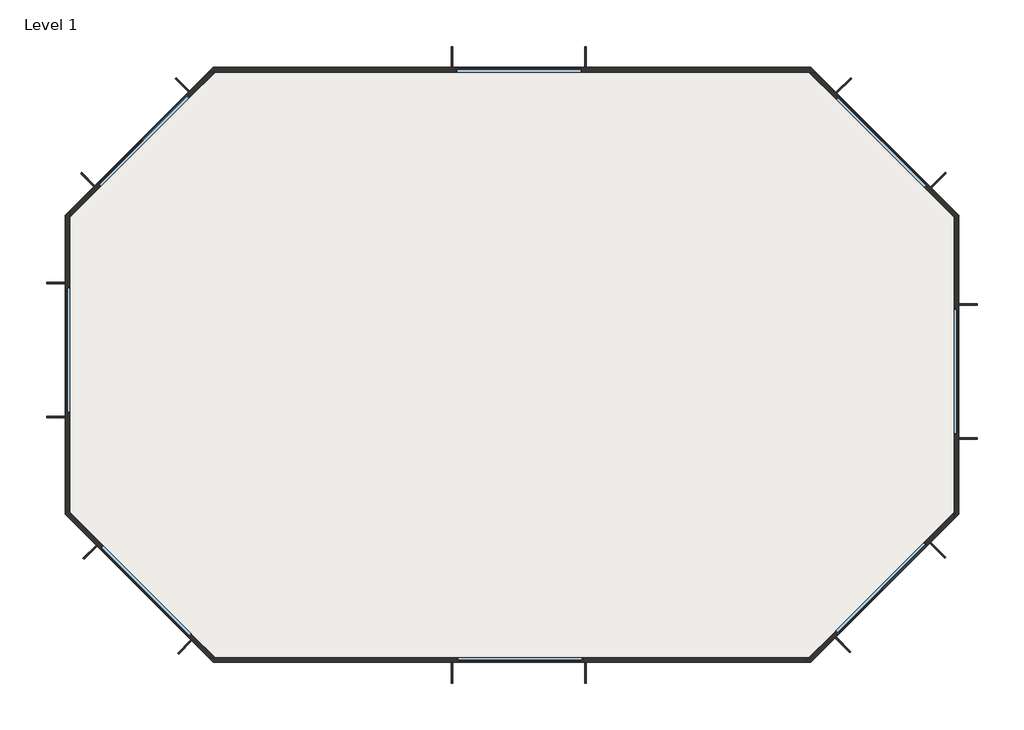
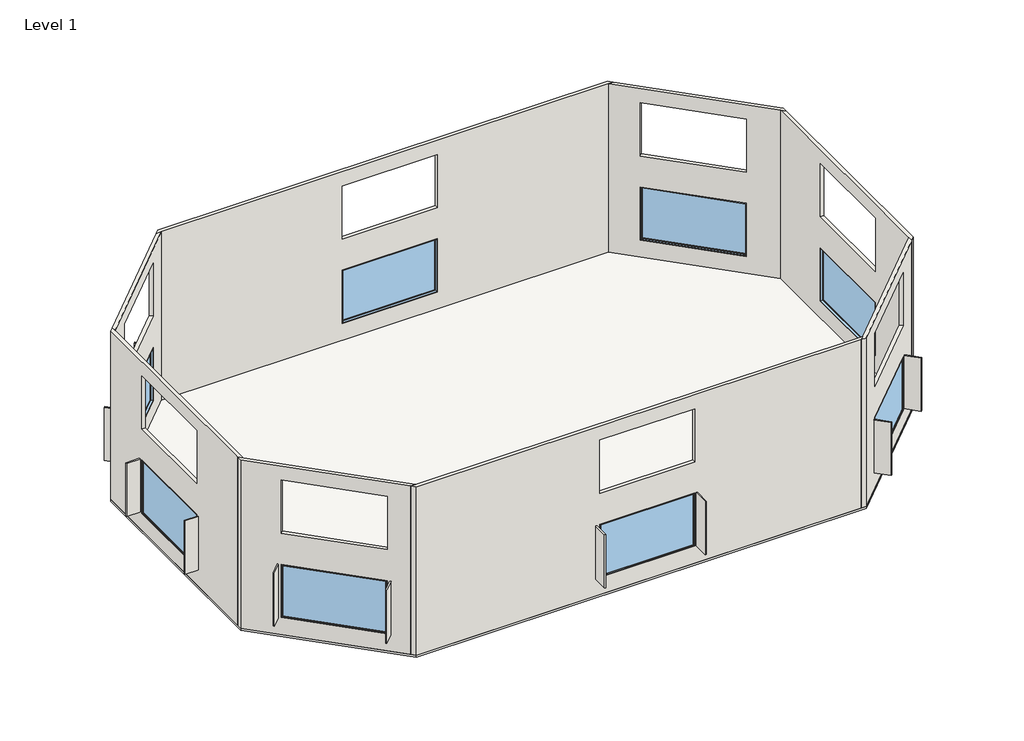
# One storey: 24 walls, 8 windows, 1 slab.
"""IFC4 building model written with IfcOpenShell, lengths in millimetres."""

import ifcopenshell
import ifcopenshell.guid

model = None  # the IFC model being written
_history = None  # IfcOwnerHistory: only IFC2X3 demands one
_inside = {}  # id of a spatial element -> (the spatial element, [elements in it])
_under = {}  # id of a project, library or spatial element -> (it, [spatial elements below it])
_declared = {}  # id of a project -> (the project, [libraries it declares])
_typed = {}  # id of a type object -> (the type object, [elements of that type])
_made_of = {}  # id of a material, layer set ... -> (it, [elements and type objects made of it])


def new_model(schema):
    """Start an empty IFC model of exactly this schema.

    Asked for "IFC4X3", IfcOpenShell would pick the latest addendum, in which some entities
    have other attributes; the version numbers below select the first issue.
    IFC2X3 requires an IfcOwnerHistory on every rooted entity: one is made here for all.
    """
    global model, _history
    if schema == "IFC4X3":
        model = ifcopenshell.file(schema_version=(4, 3, 0, 0))
    else:
        model = ifcopenshell.file(schema=schema)
    _inside.clear()
    _under.clear()
    _declared.clear()
    _typed.clear()
    _made_of.clear()
    _history = None
    if model.schema == "IFC2X3":
        org = make("IfcOrganization", Name="unknown")
        user = make(
            "IfcPersonAndOrganization",
            ThePerson=make("IfcPerson", FamilyName="unknown"),
            TheOrganization=org,
        )
        app = make(
            "IfcApplication",
            ApplicationDeveloper=org,
            Version="unknown",
            ApplicationFullName="unknown",
            ApplicationIdentifier="unknown",
        )
        _history = make(
            "IfcOwnerHistory",
            OwningUser=user,
            OwningApplication=app,
            ChangeAction="ADDED",
            CreationDate=0,
        )
    return model


def make(cls, **values):
    """One entity of the class cls with the attributes given. An attribute that is None is left unset."""
    return model.create_entity(
        cls, **{name: value for name, value in values.items() if value is not None}
    )


def rooted(cls, **values):
    """An entity with a GlobalId (a new one), such as an element, a storey or a relation."""
    return make(cls, GlobalId=ifcopenshell.guid.new(), OwnerHistory=_history, **values)


def si_unit(unit_type, name, prefix=None):
    """IfcSIUnit, for example si_unit("LENGTHUNIT", "METRE", prefix="MILLI")."""
    return make("IfcSIUnit", UnitType=unit_type, Prefix=prefix, Name=name)


def assignment(units):
    """IfcUnitAssignment: the units of a project."""
    return None if units is None else make("IfcUnitAssignment", Units=units)


def point(xyz):
    """IfcCartesianPoint."""
    return None if xyz is None else make("IfcCartesianPoint", Coordinates=xyz)


def direction(xyz):
    """IfcDirection."""
    return None if xyz is None else make("IfcDirection", DirectionRatios=xyz)


def frame(location, z_axis=None, x_axis=None):
    """IfcAxis2Placement3D, a coordinate frame: its origin and axes. An axis left out is left unset."""
    return make(
        "IfcAxis2Placement3D",
        Location=point(location),
        Axis=direction(z_axis),
        RefDirection=direction(x_axis),
    )


def origin():
    """The frame at (0, 0, 0) with its axes left unset."""
    return frame((0.0, 0.0, 0.0))


def place(relative_to, where):
    """IfcLocalPlacement: puts the frame where relative to a parent placement (None: the world)."""
    return make(
        "IfcLocalPlacement", PlacementRelTo=relative_to, RelativePlacement=where
    )


def context(
    kind, dimensions, precision=None, world=None, true_north=None, identifier=None
):
    """IfcGeometricRepresentationContext, for example the 3D "Model" context."""
    return make(
        "IfcGeometricRepresentationContext",
        ContextIdentifier=identifier,
        ContextType=kind,
        CoordinateSpaceDimension=dimensions,
        Precision=precision,
        WorldCoordinateSystem=world,
        TrueNorth=true_north,
    )


def project(units=None, contexts=None):
    """IfcProject with its units and contexts."""
    return rooted(
        "IfcProject",
        Name="project",
        RepresentationContexts=contexts,
        UnitsInContext=assignment(units),
    )


def spatial(cls, under=None, at=None, **own):
    """A site, building, storey or space (cls), placed at a placement, below another one or the project."""
    s = rooted(cls, ObjectPlacement=at, **own)
    if under is not None:
        _under.setdefault(under.id(), (under, []))[1].append(s)
    return s


def polyline(points):
    """IfcPolyline through the points."""
    return make("IfcPolyline", Points=[point(p) for p in points])


def outline(outer, holes=None, kind="AREA"):
    """IfcArbitraryClosedProfileDef: a profile drawn as a closed curve; with holes, ...WithVoids."""
    if holes is None:
        return make("IfcArbitraryClosedProfileDef", ProfileType=kind, OuterCurve=outer)
    return make(
        "IfcArbitraryProfileDefWithVoids",
        ProfileType=kind,
        OuterCurve=outer,
        InnerCurves=holes,
    )


def extrude(swept, where, along, depth):
    """IfcExtrudedAreaSolid: the profile swept, set in the frame where, extruded along a direction by depth."""
    return make(
        "IfcExtrudedAreaSolid",
        SweptArea=swept,
        Position=where,
        ExtrudedDirection=direction(along),
        Depth=depth,
    )


def faces_of(points, faces, orient=None, outer=None):
    """IfcFace entities. A face is a list of loops; a loop is a list of indices into points, from 0.

    orient and outer hold one flag for each loop. By default every Orientation is true, the
    first loop of a face is its IfcFaceOuterBound and the others are IfcFaceBound.
    """
    made = []
    for i, loops in enumerate(faces):
        bounds = []
        for j, loop in enumerate(loops):
            is_outer = j == 0 if outer is None else outer[i][j]
            bounds.append(
                make(
                    "IfcFaceOuterBound" if is_outer else "IfcFaceBound",
                    Bound=make("IfcPolyLoop", Polygon=[points[k] for k in loop]),
                    Orientation=True if orient is None else orient[i][j],
                )
            )
        made.append(make("IfcFace", Bounds=bounds))
    return made


def faceted_brep(points, faces, orient=None, outer=None, voids=None):
    """IfcFacetedBrep: a solid bounded by flat faces; with voids (closed shells), ...WithVoids."""
    shared = [point(p) for p in points]
    hull = make("IfcClosedShell", CfsFaces=faces_of(shared, faces, orient, outer))
    if voids is None:
        return make("IfcFacetedBrep", Outer=hull)
    return make(
        "IfcFacetedBrepWithVoids",
        Outer=hull,
        Voids=[
            make(cls, CfsFaces=faces_of(shared, fs, o, b)) for cls, fs, o, b in voids
        ],
    )


def shape(context_of_items, identifier, shape_type, items):
    """IfcShapeRepresentation: the items that make up one representation, for example the "Body"."""
    return make(
        "IfcShapeRepresentation",
        ContextOfItems=context_of_items,
        RepresentationIdentifier=identifier,
        RepresentationType=shape_type,
        Items=items,
    )


def source(mapping_origin, context_of_items, identifier, shape_type, items):
    """IfcRepresentationMap: a shape defined once, which mapped items show again and again."""
    return make(
        "IfcRepresentationMap",
        MappingOrigin=mapping_origin,
        MappedRepresentation=shape(context_of_items, identifier, shape_type, items),
    )


def transform(
    local_origin,
    x_axis=None,
    y_axis=None,
    z_axis=None,
    scale=None,
    scale2=None,
    scale3=None,
    uniform=True,
):
    """IfcCartesianTransformationOperator3D, or its non-uniform kind. x_axis, y_axis, z_axis: its Axis1, 2, 3."""
    if uniform:
        return make(
            "IfcCartesianTransformationOperator3D",
            Axis1=direction(x_axis),
            Axis2=direction(y_axis),
            LocalOrigin=point(local_origin),
            Scale=scale,
            Axis3=direction(z_axis),
        )
    return make(
        "IfcCartesianTransformationOperator3DnonUniform",
        Axis1=direction(x_axis),
        Axis2=direction(y_axis),
        LocalOrigin=point(local_origin),
        Scale=scale,
        Axis3=direction(z_axis),
        Scale2=scale2,
        Scale3=scale3,
    )


def mapped(mapping_source, mapping_target):
    """IfcMappedItem: shows the shape of a source again, moved by a transform."""
    return make(
        "IfcMappedItem", MappingSource=mapping_source, MappingTarget=mapping_target
    )


def made_of(thing, what):
    """Note that an element or type object is made of a material, layer set ...; save() writes the relation."""
    if what is not None:
        _made_of.setdefault(what.id(), (what, []))[1].append(thing)
    return thing


def element(
    cls,
    number,
    at=None,
    inside=None,
    cuts=None,
    type_object=None,
    material=None,
    context=None,
    identifier="Body",
    shape_type=None,
    held_by="IfcProductDefinitionShape",
    body=None,
    shapes=None,
    **own,
):
    """One element of the class cls, such as IfcWall. Its Tag is "e" and its number.

    at: its placement. inside: the storey or other place that contains it. cuts: it is an
    opening in that element (IfcRelVoidsElement). A single representation is given by context,
    identifier, shape_type and body (its items); several are given by shapes. held_by: the class
    of the entity that holds the representations. save() writes the other relations.
    """
    e = rooted(cls, Tag="e%d" % number, ObjectPlacement=at, **own)
    if body is not None:
        shapes = [shape(context, identifier, shape_type, body)]
    if shapes is not None:
        e.Representation = make(held_by, Representations=shapes)
    if inside is not None:
        _inside.setdefault(inside.id(), (inside, []))[1].append(e)
    if cuts is not None:
        rooted(
            "IfcRelVoidsElement", RelatingBuildingElement=cuts, RelatedOpeningElement=e
        )
    if type_object is not None:
        _typed.setdefault(type_object.id(), (type_object, []))[1].append(e)
    return made_of(e, material)


def aggregate(whole, parts):
    """IfcRelAggregates: a whole, such as a stair, and the parts it consists of."""
    return rooted("IfcRelAggregates", RelatingObject=whole, RelatedObjects=parts)


def save(model, path):
    """Write the relations noted so far, then the file.

    IfcRelAggregates (storeys below a building ...), IfcRelContainedInSpatialStructure (elements
    in a storey), IfcRelDefinesByType, IfcRelAssociatesMaterial and IfcRelDeclares: one each for
    every whole, place, type object, material and project.
    """
    for whole, parts in _under.values():
        aggregate(whole, parts)
    for where, things in _inside.values():
        rooted(
            "IfcRelContainedInSpatialStructure",
            RelatedElements=things,
            RelatingStructure=where,
        )
    for kind, things in _typed.values():
        rooted("IfcRelDefinesByType", RelatedObjects=things, RelatingType=kind)
    for what, things in _made_of.values():
        rooted("IfcRelAssociatesMaterial", RelatedObjects=things, RelatingMaterial=what)
    for by, libraries in _declared.values():
        rooted("IfcRelDeclares", RelatingContext=by, RelatedDefinitions=libraries)
    model.write(path)


def m_fixed_2500x_4228mm_fd5e51e7(model_context):
    return source(origin(), model_context, "Body", "SweptSolid", [
        extrude(outline(polyline([(-2050.8, 54.2), (2050.8, 54.2), (2050.8, 42.2), (-2050.8, 42.2), (-2050.8, 54.2)])), frame((0.0, 0.0, 368.0), z_axis=(0.0, 0.0, 1.0), x_axis=(1.0, 0.0, 0.0)), (0.0, 0.0, 1.0), 2374.0),
        extrude(outline(polyline([(2786.0, -2094.8), (324.0, -2094.8), (324.0, 2094.8), (2786.0, 2094.8), (2786.0, -2094.8)]), holes=[polyline([(2742.0, -2050.8), (2742.0, 2050.8), (368.0, 2050.8), (368.0, -2050.8), (2742.0, -2050.8)])]), frame((0.0, 26.2, 0.0), z_axis=(0.0, 1.0, 0.0), x_axis=(0.0, 0.0, 1.0)), (0.0, 0.0, 1.0), 44.0),
        extrude(outline(polyline([(2805.0, -2113.8), (305.0, -2113.8), (305.0, 2113.8), (2805.0, 2113.8), (2805.0, -2113.8)]), holes=[polyline([(2786.0, -2094.8), (2786.0, 2094.8), (324.0, 2094.8), (324.0, -2094.8), (2786.0, -2094.8)])]), frame((0.0, 26.2, 0.0), z_axis=(0.0, 1.0, 0.0), x_axis=(0.0, 0.0, 1.0)), (0.0, 0.0, 1.0), 63.0),
        extrude(outline(polyline([(2805.0, -2113.8), (305.0, -2113.8), (305.0, 2113.8), (2805.0, 2113.8), (2805.0, -2113.8)]), holes=[polyline([(2773.0, -2081.8), (2773.0, 2081.8), (337.0, 2081.8), (337.0, -2081.8), (2773.0, -2081.8)])]), frame((0.0, -63.2, 0.0), z_axis=(0.0, 1.0, 0.0), x_axis=(0.0, 0.0, 1.0)), (0.0, 0.0, 1.0), 89.4),
    ])


model = new_model("IFC4")

# Units and contexts
model_context = context("Model", 3, world=origin())
ifc_project = project(units=[si_unit("LENGTHUNIT", "METRE", prefix="MILLI")], contexts=[model_context])

# Site, building, storey
site = spatial("IfcSite", under=ifc_project)
building = spatial("IfcBuilding", under=site)
storey = spatial("IfcBuildingStorey", under=building, Name="Level 1", Elevation=0.0)

# Slab
placement = place(None, origin())
element("IfcSlab", 1, ObjectType="Generic Floor - 100mm", at=placement, inside=storey, context=model_context, shape_type="SweptSolid", body=[
    extrude(outline(polyline([(10639.2142415, 11296.9802217), (30639.2142415, 11296.9802217), (35588.9617098, 6347.2327534), (35588.9617098, -3652.7672466), (30639.2142415, -8602.5147149), (10639.2142415, -8602.5147149), (5689.4667732, -3652.7672466), (5689.4667732, 6347.2327534), (10639.2142415, 11296.9802217)])), frame((0.0, 0.0, -100.0), z_axis=(0.0, 0.0, 1.0), x_axis=(1.0, 0.0, 0.0)), (0.0, 0.0, 1.0), 100.0),
])

# Walls
element("IfcWall", 2, ObjectType="Generic - 152.4mm", at=placement, inside=storey, context=model_context, shape_type="Brep", body=[
    faceted_brep([(10486.8142415, 11144.5802217, 0.0), (10702.3403884, 11144.5802217, 0.0), (30576.0880946, 11144.5802217, 0.0), (30791.6142415, 11144.5802217, 0.0), (30791.6142415, 11144.5802217, 7924.8), (30576.0880946, 11144.5802217, 7924.8), (10702.3403884, 11144.5802217, 7924.8), (10486.8142415, 11144.5802217, 7924.8), (18752.7836697, 11144.5802217, 4762.4), (18752.7836697, 11144.5802217, 7262.4), (22980.3836697, 11144.5802217, 7262.4), (22980.3836697, 11144.5802217, 4762.4), (18752.7836697, 11144.5802217, 800.0), (18752.7836697, 11144.5802217, 3300.0), (22980.3836697, 11144.5802217, 3300.0), (22980.3836697, 11144.5802217, 800.0), (10639.2142415, 11296.9802217, 0.0), (10639.2142415, 11296.9802217, 7924.8), (30639.2142415, 11296.9802217, 7924.8), (30639.2142415, 11296.9802217, 0.0), (18752.7836697, 11296.9802217, 4762.4), (22980.3836697, 11296.9802217, 4762.4), (22980.3836697, 11296.9802217, 7262.4), (18752.7836697, 11296.9802217, 7262.4), (18752.7836697, 11296.9802217, 800.0), (22980.3836697, 11296.9802217, 800.0), (22980.3836697, 11296.9802217, 3300.0), (18752.7836697, 11296.9802217, 3300.0)], [[[0, 1, 2, 3, 4, 5, 6, 7], [8, 9, 10, 11], [12, 13, 14, 15]], [[16, 17, 18, 19], [20, 21, 22, 23], [24, 25, 26, 27]], [[3, 2, 1, 0, 16, 19]], [[7, 6, 5, 4, 18, 17]], [[4, 3, 19, 18]], [[0, 7, 17, 16]], [[9, 8, 20, 23]], [[10, 9, 23, 22]], [[11, 10, 22, 21]], [[8, 11, 21, 20]], [[13, 12, 24, 27]], [[14, 13, 27, 26]], [[15, 14, 26, 25]], [[12, 15, 25, 24]]]),
])
element("IfcWall", 3, ObjectType="Generic - 152.4mm", at=placement, inside=storey, context=model_context, shape_type="Brep", body=[
    faceted_brep([(30576.0880946, 11144.5802217, 0.0), (35436.5617098, 6284.1066065, 0.0), (35588.9617098, 6131.7066065, 0.0), (35588.9617098, 6131.7066065, 7924.8), (35436.5617098, 6284.1066065, 7924.8), (30576.0880946, 11144.5802217, 7924.8), (31471.8841839, 10248.7841324, 4762.4), (31471.8841839, 10248.7841324, 7262.4), (34461.2488121, 7259.4195042, 7262.4), (34461.2488121, 7259.4195042, 4762.4), (31471.8841839, 10248.7841324, 800.0), (31471.8841839, 10248.7841324, 3300.0), (34461.2488121, 7259.4195042, 3300.0), (34461.2488121, 7259.4195042, 800.0), (30791.6142415, 11144.5802217, 0.0), (30791.6142415, 11144.5802217, 7924.8), (35588.9617098, 6347.2327534, 7924.8), (35588.9617098, 6347.2327534, 0.0), (31579.6472574, 10356.5472058, 4762.4), (34569.0118855, 7367.1825777, 4762.4), (34569.0118855, 7367.1825777, 7262.4), (31579.6472574, 10356.5472058, 7262.4), (31579.6472574, 10356.5472058, 800.0), (34569.0118855, 7367.1825777, 800.0), (34569.0118855, 7367.1825777, 3300.0), (31579.6472574, 10356.5472058, 3300.0)], [[[0, 1, 2, 3, 4, 5], [6, 7, 8, 9], [10, 11, 12, 13]], [[14, 15, 16, 17], [18, 19, 20, 21], [22, 23, 24, 25]], [[2, 1, 0, 14, 17]], [[5, 4, 3, 16, 15]], [[0, 5, 15, 14]], [[3, 2, 17, 16]], [[7, 6, 18, 21]], [[8, 7, 21, 20]], [[9, 8, 20, 19]], [[6, 9, 19, 18]], [[11, 10, 22, 25]], [[12, 11, 25, 24]], [[13, 12, 24, 23]], [[10, 13, 23, 22]]]),
])
element("IfcWall", 4, ObjectType="Generic - 152.4mm", at=placement, inside=storey, context=model_context, shape_type="Brep", body=[
    faceted_brep([(35436.5617098, 6284.1066065, 0.0), (35436.5617098, -3589.6410997, 0.0), (35436.5617098, -3805.1672466, 0.0), (35436.5617098, -3805.1672466, 7924.8), (35436.5617098, -3589.6410997, 7924.8), (35436.5617098, 6284.1066065, 7924.8), (35436.5617098, 3236.2401206, 4762.4), (35436.5617098, 3236.2401206, 7262.4), (35436.5617098, -991.3598794, 7262.4), (35436.5617098, -991.3598794, 4762.4), (35436.5617098, 3236.2401206, 800.0), (35436.5617098, 3236.2401206, 3300.0), (35436.5617098, -991.3598794, 3300.0), (35436.5617098, -991.3598794, 800.0), (35588.9617098, 6131.7066065, 0.0), (35588.9617098, 6131.7066065, 7924.8), (35588.9617098, -3652.7672466, 7924.8), (35588.9617098, -3652.7672466, 0.0), (35588.9617098, 3236.2401206, 4762.4), (35588.9617098, -991.3598794, 4762.4), (35588.9617098, -991.3598794, 7262.4), (35588.9617098, 3236.2401206, 7262.4), (35588.9617098, 3236.2401206, 800.0), (35588.9617098, -991.3598794, 800.0), (35588.9617098, -991.3598794, 3300.0), (35588.9617098, 3236.2401206, 3300.0)], [[[0, 1, 2, 3, 4, 5], [6, 7, 8, 9], [10, 11, 12, 13]], [[14, 15, 16, 17], [18, 19, 20, 21], [22, 23, 24, 25]], [[2, 1, 0, 14, 17]], [[5, 4, 3, 16, 15]], [[0, 5, 15, 14]], [[3, 2, 17, 16]], [[7, 6, 18, 21]], [[8, 7, 21, 20]], [[9, 8, 20, 19]], [[6, 9, 19, 18]], [[11, 10, 22, 25]], [[12, 11, 25, 24]], [[13, 12, 24, 23]], [[10, 13, 23, 22]]]),
])
element("IfcWall", 5, ObjectType="Generic - 152.4mm", at=placement, inside=storey, context=model_context, shape_type="Brep", body=[
    faceted_brep([(35436.5617098, -3589.6410997, 0.0), (30576.0880946, -8450.1147149, 0.0), (30423.6880946, -8602.5147149, 0.0), (30423.6880946, -8602.5147149, 7924.8), (30576.0880946, -8450.1147149, 7924.8), (35436.5617098, -3589.6410997, 7924.8), (34437.5479697, -4588.6548399, 4762.4), (34437.5479697, -4588.6548399, 7262.4), (31448.1833416, -7578.019468, 7262.4), (31448.1833416, -7578.019468, 4762.4), (34437.5479697, -4588.6548399, 800.0), (34437.5479697, -4588.6548399, 3300.0), (31448.1833416, -7578.019468, 3300.0), (31448.1833416, -7578.019468, 800.0), (30639.2142415, -8602.5147149, 0.0), (35436.5617098, -3805.1672466, 0.0), (35436.5617098, -3805.1672466, 7924.8), (30639.2142415, -8602.5147149, 7924.8), (34545.3110432, -4696.4179133, 7262.4), (34545.3110432, -4696.4179133, 4762.4), (31555.946415, -7685.7825415, 4762.4), (31555.946415, -7685.7825415, 7262.4), (34545.3110432, -4696.4179133, 3300.0), (34545.3110432, -4696.4179133, 800.0), (31555.946415, -7685.7825415, 800.0), (31555.946415, -7685.7825415, 3300.0)], [[[0, 1, 2, 3, 4, 5], [6, 7, 8, 9], [10, 11, 12, 13]], [[14, 15, 16, 17], [18, 19, 20, 21], [22, 23, 24, 25]], [[2, 1, 0, 15, 14]], [[5, 4, 3, 17, 16]], [[0, 5, 16, 15]], [[3, 2, 14, 17]], [[6, 19, 18, 7]], [[7, 18, 21, 8]], [[8, 21, 20, 9]], [[19, 6, 9, 20]], [[11, 10, 23, 22]], [[12, 11, 22, 25]], [[13, 12, 25, 24]], [[10, 13, 24, 23]]]),
])
element("IfcWall", 6, ObjectType="Generic - 152.4mm", at=placement, inside=storey, context=model_context, shape_type="Brep", body=[
    faceted_brep([(30576.0880946, -8450.1147149, 0.0), (10702.3403884, -8450.1147149, 0.0), (10486.8142415, -8450.1147149, 0.0), (10486.8142415, -8450.1147149, 7924.8), (10702.3403884, -8450.1147149, 7924.8), (30576.0880946, -8450.1147149, 7924.8), (23020.9791073, -8450.1147149, 4762.4), (23020.9791073, -8450.1147149, 7262.4), (18793.3791073, -8450.1147149, 7262.4), (18793.3791073, -8450.1147149, 4762.4), (23020.9791073, -8450.1147149, 800.0), (23020.9791073, -8450.1147149, 3300.0), (18793.3791073, -8450.1147149, 3300.0), (18793.3791073, -8450.1147149, 800.0), (30423.6880946, -8602.5147149, 0.0), (30423.6880946, -8602.5147149, 7924.8), (10639.2142415, -8602.5147149, 7924.8), (10639.2142415, -8602.5147149, 0.0), (23020.9791073, -8602.5147149, 4762.4), (18793.3791073, -8602.5147149, 4762.4), (18793.3791073, -8602.5147149, 7262.4), (23020.9791073, -8602.5147149, 7262.4), (23020.9791073, -8602.5147149, 800.0), (18793.3791073, -8602.5147149, 800.0), (18793.3791073, -8602.5147149, 3300.0), (23020.9791073, -8602.5147149, 3300.0)], [[[0, 1, 2, 3, 4, 5], [6, 7, 8, 9], [10, 11, 12, 13]], [[14, 15, 16, 17], [18, 19, 20, 21], [22, 23, 24, 25]], [[2, 1, 0, 14, 17]], [[5, 4, 3, 16, 15]], [[0, 5, 15, 14]], [[3, 2, 17, 16]], [[7, 6, 18, 21]], [[8, 7, 21, 20]], [[9, 8, 20, 19]], [[6, 9, 19, 18]], [[11, 10, 22, 25]], [[12, 11, 25, 24]], [[13, 12, 24, 23]], [[10, 13, 23, 22]]]),
])
element("IfcWall", 7, ObjectType="Generic - 152.4mm", at=placement, inside=storey, context=model_context, shape_type="Brep", body=[
    faceted_brep([(10702.3403884, -8450.1147149, 0.0), (5841.8667732, -3589.6410997, 0.0), (5689.4667732, -3437.2410997, 0.0), (5689.4667732, -3437.2410997, 7924.8), (5841.8667732, -3589.6410997, 7924.8), (10702.3403884, -8450.1147149, 7924.8), (9927.9208562, -7675.6951827, 4762.4), (9927.9208562, -7675.6951827, 7262.4), (6938.556228, -4686.3305545, 7262.4), (6938.556228, -4686.3305545, 4762.4), (9927.9208562, -7675.6951827, 800.0), (9927.9208562, -7675.6951827, 3300.0), (6938.556228, -4686.3305545, 3300.0), (6938.556228, -4686.3305545, 800.0), (10486.8142415, -8450.1147149, 0.0), (10486.8142415, -8450.1147149, 7924.8), (5689.4667732, -3652.7672466, 7924.8), (5689.4667732, -3652.7672466, 0.0), (9820.1577827, -7783.4582561, 4762.4), (6830.7931546, -4794.093628, 4762.4), (6830.7931546, -4794.093628, 7262.4), (9820.1577827, -7783.4582561, 7262.4), (9820.1577827, -7783.4582561, 800.0), (6830.7931546, -4794.093628, 800.0), (6830.7931546, -4794.093628, 3300.0), (9820.1577827, -7783.4582561, 3300.0)], [[[0, 1, 2, 3, 4, 5], [6, 7, 8, 9], [10, 11, 12, 13]], [[14, 15, 16, 17], [18, 19, 20, 21], [22, 23, 24, 25]], [[2, 1, 0, 14, 17]], [[5, 4, 3, 16, 15]], [[0, 5, 15, 14]], [[3, 2, 17, 16]], [[7, 6, 18, 21]], [[8, 7, 21, 20]], [[9, 8, 20, 19]], [[6, 9, 19, 18]], [[11, 10, 22, 25]], [[12, 11, 25, 24]], [[13, 12, 24, 23]], [[10, 13, 23, 22]]]),
])
element("IfcWall", 8, ObjectType="Generic - 152.4mm", at=placement, inside=storey, context=model_context, shape_type="Brep", body=[
    faceted_brep([(5841.8667732, -3589.6410997, 0.0), (5841.8667732, 6284.1066065, 0.0), (5841.8667732, 6499.6327534, 0.0), (5841.8667732, 6499.6327534, 7924.8), (5841.8667732, 6284.1066065, 7924.8), (5841.8667732, -3589.6410997, 7924.8), (5841.8667732, -270.991266, 4762.4), (5841.8667732, -270.991266, 7262.4), (5841.8667732, 3956.608734, 7262.4), (5841.8667732, 3956.608734, 4762.4), (5841.8667732, -270.991266, 800.0), (5841.8667732, -270.991266, 3300.0), (5841.8667732, 3956.608734, 3300.0), (5841.8667732, 3956.608734, 800.0), (5689.4667732, -3437.2410997, 0.0), (5689.4667732, -3437.2410997, 7924.8), (5689.4667732, 6347.2327534, 7924.8), (5689.4667732, 6347.2327534, 0.0), (5689.4667732, -270.991266, 4762.4), (5689.4667732, 3956.608734, 4762.4), (5689.4667732, 3956.608734, 7262.4), (5689.4667732, -270.991266, 7262.4), (5689.4667732, -270.991266, 800.0), (5689.4667732, 3956.608734, 800.0), (5689.4667732, 3956.608734, 3300.0), (5689.4667732, -270.991266, 3300.0)], [[[0, 1, 2, 3, 4, 5], [6, 7, 8, 9], [10, 11, 12, 13]], [[14, 15, 16, 17], [18, 19, 20, 21], [22, 23, 24, 25]], [[2, 1, 0, 14, 17]], [[5, 4, 3, 16, 15]], [[0, 5, 15, 14]], [[3, 2, 17, 16]], [[7, 6, 18, 21]], [[8, 7, 21, 20]], [[9, 8, 20, 19]], [[6, 9, 19, 18]], [[11, 10, 22, 25]], [[12, 11, 25, 24]], [[13, 12, 24, 23]], [[10, 13, 23, 22]]]),
])
element("IfcWall", 9, ObjectType="Generic - 152.4mm", at=placement, inside=storey, context=model_context, shape_type="Brep", body=[
    faceted_brep([(5841.8667732, 6284.1066065, 0.0), (10702.3403884, 11144.5802217, 0.0), (10702.3403884, 11144.5802217, 7924.8), (5841.8667732, 6284.1066065, 7924.8), (6863.3827465, 7305.6225798, 4762.4), (6863.3827465, 7305.6225798, 7262.4), (9852.7473747, 10294.9872079, 7262.4), (9852.7473747, 10294.9872079, 4762.4), (6863.3827465, 7305.6225798, 800.0), (6863.3827465, 7305.6225798, 3300.0), (9852.7473747, 10294.9872079, 3300.0), (9852.7473747, 10294.9872079, 800.0), (5841.8667732, 6499.6327534, 0.0), (5841.8667732, 6499.6327534, 7924.8), (10486.8142415, 11144.5802217, 7924.8), (10486.8142415, 11144.5802217, 0.0), (6755.6196731, 7413.3856532, 4762.4), (9744.9843012, 10402.7502814, 4762.4), (9744.9843012, 10402.7502814, 7262.4), (6755.6196731, 7413.3856532, 7262.4), (6755.6196731, 7413.3856532, 800.0), (9744.9843012, 10402.7502814, 800.0), (9744.9843012, 10402.7502814, 3300.0), (6755.6196731, 7413.3856532, 3300.0)], [[[0, 1, 2, 3], [4, 5, 6, 7], [8, 9, 10, 11]], [[12, 13, 14, 15], [16, 17, 18, 19], [20, 21, 22, 23]], [[1, 0, 12, 15]], [[3, 2, 14, 13]], [[0, 3, 13, 12]], [[2, 1, 15, 14]], [[5, 4, 16, 19]], [[6, 5, 19, 18]], [[7, 6, 18, 17]], [[4, 7, 17, 16]], [[9, 8, 20, 23]], [[10, 9, 23, 22]], [[11, 10, 22, 21]], [[8, 11, 21, 20]]]),
])
element("IfcWall", 10, ObjectType="Generic - Shading", at=placement, inside=storey, context=model_context, shape_type="SweptSolid", body=[
    extrude(outline(polyline([(18602.7836697, -9302.5147149), (18602.7836697, -8602.5147149), (18652.7836697, -8602.5147149), (18652.7836697, -9302.5147149), (18602.7836697, -9302.5147149)])), frame((0.0, 0.0, 800.0), z_axis=(0.0, 0.0, 1.0), x_axis=(1.0, 0.0, 0.0)), (0.0, 0.0, 1.0), 2500.0),
])
element("IfcWall", 11, ObjectType="Generic - Shading", at=placement, inside=storey, context=model_context, shape_type="SweptSolid", body=[
    extrude(outline(polyline([(23080.3836697, -9302.5147149), (23080.3836697, -8602.5147149), (23130.3836697, -8602.5147149), (23130.3836697, -9302.5147149), (23080.3836697, -9302.5147149)])), frame((0.0, 0.0, 800.0), z_axis=(0.0, 0.0, 1.0), x_axis=(1.0, 0.0, 0.0)), (0.0, 0.0, 1.0), 2500.0),
])
element("IfcWall", 12, ObjectType="Generic - Shading", at=placement, inside=storey, context=model_context, shape_type="SweptSolid", body=[
    extrude(outline(polyline([(18652.7836697, 11996.9802217), (18652.7836697, 11296.9802217), (18602.7836697, 11296.9802217), (18602.7836697, 11996.9802217), (18652.7836697, 11996.9802217)])), frame((0.0, 0.0, 800.0), z_axis=(0.0, 0.0, 1.0), x_axis=(1.0, 0.0, 0.0)), (0.0, 0.0, 1.0), 2500.0),
])
element("IfcWall", 13, ObjectType="Generic - Shading", at=placement, inside=storey, context=model_context, shape_type="SweptSolid", body=[
    extrude(outline(polyline([(23130.3836697, 11996.9802217), (23130.3836697, 11296.9802217), (23080.3836697, 11296.9802217), (23080.3836697, 11996.9802217), (23130.3836697, 11996.9802217)])), frame((0.0, 0.0, 800.0), z_axis=(0.0, 0.0, 1.0), x_axis=(1.0, 0.0, 0.0)), (0.0, 0.0, 1.0), 2500.0),
])
element("IfcWall", 14, ObjectType="Generic - Shading", at=placement, inside=storey, context=model_context, shape_type="SweptSolid", body=[
    extrude(outline(polyline([(32003.1901519, 10922.602081), (31508.391267, 10427.8031962), (31473.035928, 10463.1585352), (31967.8348129, 10957.9574201), (32003.1901519, 10922.602081)])), frame((0.0, 0.0, 800.0), z_axis=(0.0, 0.0, 1.0), x_axis=(1.0, 0.0, 0.0)), (0.0, 0.0, 1.0), 2500.0),
])
element("IfcWall", 15, ObjectType="Generic - Shading", at=placement, inside=storey, context=model_context, shape_type="SweptSolid", body=[
    extrude(outline(polyline([(35169.8767876, 7755.9154454), (34675.0779027, 7261.1165605), (34639.7225636, 7296.4718995), (35134.5214485, 7791.2707844), (35169.8767876, 7755.9154454)])), frame((0.0, 0.0, 800.0), z_axis=(0.0, 0.0, 1.0), x_axis=(1.0, 0.0, 0.0)), (0.0, 0.0, 1.0), 2500.0),
])
element("IfcWall", 16, ObjectType="Generic - Shading", at=placement, inside=storey, context=model_context, shape_type="SweptSolid", body=[
    extrude(outline(polyline([(31944.1339705, -8287.1927558), (31449.3350856, -7792.3938709), (31484.6904247, -7757.0385318), (31979.4893096, -8251.8374167), (31944.1339705, -8287.1927558)])), frame((0.0, 0.0, 800.0), z_axis=(0.0, 0.0, 1.0), x_axis=(1.0, 0.0, 0.0)), (0.0, 0.0, 1.0), 2500.0),
])
element("IfcWall", 17, ObjectType="Generic - Shading", at=placement, inside=storey, context=model_context, shape_type="SweptSolid", body=[
    extrude(outline(polyline([(35110.8206062, -5120.5061201), (34616.0217213, -4625.7072352), (34651.3770603, -4590.3518961), (35146.1759452, -5085.150781), (35110.8206062, -5120.5061201)])), frame((0.0, 0.0, 800.0), z_axis=(0.0, 0.0, 1.0), x_axis=(1.0, 0.0, 0.0)), (0.0, 0.0, 1.0), 2500.0),
])
element("IfcWall", 18, ObjectType="Generic - Shading", at=placement, inside=storey, context=model_context, shape_type="SweptSolid", body=[
    extrude(outline(polyline([(9410.5024205, 10950.4548209), (9851.5956306, 10509.3616108), (9816.2402916, 10474.0062717), (9375.1470815, 10915.0994818), (9410.5024205, 10950.4548209)])), frame((0.0, 0.0, 800.0), z_axis=(0.0, 0.0, 1.0), x_axis=(1.0, 0.0, 0.0)), (0.0, 0.0, 1.0), 2500.0),
])
element("IfcWall", 19, ObjectType="Generic - Shading", at=placement, inside=storey, context=model_context, shape_type="SweptSolid", body=[
    extrude(outline(polyline([(6243.8157849, 7783.7681852), (6684.908995, 7342.6749751), (6649.5536559, 7307.319636), (6208.4604458, 7748.4128461), (6243.8157849, 7783.7681852)])), frame((0.0, 0.0, 800.0), z_axis=(0.0, 0.0, 1.0), x_axis=(1.0, 0.0, 0.0)), (0.0, 0.0, 1.0), 2500.0),
])
element("IfcWall", 20, ObjectType="Generic - Shading", at=placement, inside=storey, context=model_context, shape_type="SweptSolid", body=[
    extrude(outline(polyline([(9450.3205629, -8295.8074566), (9891.413773, -7854.7142465), (9926.7691121, -7890.0695855), (9485.675902, -8331.1627956), (9450.3205629, -8295.8074566)])), frame((0.0, 0.0, 800.0), z_axis=(0.0, 0.0, 1.0), x_axis=(1.0, 0.0, 0.0)), (0.0, 0.0, 1.0), 2500.0),
])
element("IfcWall", 21, ObjectType="Generic - Shading", at=placement, inside=storey, context=model_context, shape_type="SweptSolid", body=[
    extrude(outline(polyline([(6283.6339273, -5129.1208209), (6724.7271374, -4688.0276108), (6760.0824764, -4723.3829499), (6318.9892663, -5164.47616), (6283.6339273, -5129.1208209)])), frame((0.0, 0.0, 800.0), z_axis=(0.0, 0.0, 1.0), x_axis=(1.0, 0.0, 0.0)), (0.0, 0.0, 1.0), 2500.0),
])
element("IfcWall", 22, ObjectType="Generic - Shading", at=placement, inside=storey, context=model_context, shape_type="SweptSolid", body=[
    extrude(outline(polyline([(36212.7617098, -1141.3598794), (35588.9617098, -1141.3598794), (35588.9617098, -1091.3598794), (36212.7617098, -1091.3598794), (36212.7617098, -1141.3598794)])), frame((0.0, 0.0, 800.0), z_axis=(0.0, 0.0, 1.0), x_axis=(1.0, 0.0, 0.0)), (0.0, 0.0, 1.0), 2500.0),
])
element("IfcWall", 23, ObjectType="Generic - Shading", at=placement, inside=storey, context=model_context, shape_type="SweptSolid", body=[
    extrude(outline(polyline([(36212.7617098, 3336.2401206), (35588.9617098, 3336.2401206), (35588.9617098, 3386.2401206), (36212.7617098, 3386.2401206), (36212.7617098, 3336.2401206)])), frame((0.0, 0.0, 800.0), z_axis=(0.0, 0.0, 1.0), x_axis=(1.0, 0.0, 0.0)), (0.0, 0.0, 1.0), 2500.0),
])
element("IfcWall", 24, ObjectType="Generic - Shading", at=placement, inside=storey, context=model_context, shape_type="SweptSolid", body=[
    extrude(outline(polyline([(5065.6667732, -370.991266), (5689.4667732, -370.991266), (5689.4667732, -420.991266), (5065.6667732, -420.991266), (5065.6667732, -370.991266)])), frame((0.0, 0.0, 800.0), z_axis=(0.0, 0.0, 1.0), x_axis=(1.0, 0.0, 0.0)), (0.0, 0.0, 1.0), 2500.0),
])
element("IfcWall", 25, ObjectType="Generic - Shading", at=placement, inside=storey, context=model_context, shape_type="SweptSolid", body=[
    extrude(outline(polyline([(5065.6667732, 4106.608734), (5689.4667732, 4106.608734), (5689.4667732, 4056.608734), (5065.6667732, 4056.608734), (5065.6667732, 4106.608734)])), frame((0.0, 0.0, 800.0), z_axis=(0.0, 0.0, 1.0), x_axis=(1.0, 0.0, 0.0)), (0.0, 0.0, 1.0), 2500.0),
])

# Windows
m_fixed_2500x_4228mm_shape = m_fixed_2500x_4228mm_fd5e51e7(model_context)
element("IfcWindow", 26, ObjectType="M_Fixed : 2500X 4228mm", at=placement, inside=storey, context=model_context, shape_type="MappedRepresentation", body=[
    mapped(m_fixed_2500x_4228mm_shape, transform((20907.1791073, -8513.3147149, 495.0), x_axis=(-1.0, 0.0, 0.0), y_axis=(0.0, -1.0, 0.0), z_axis=(0.0, 0.0, 1.0))),
])
element("IfcWindow", 27, ObjectType="M_Fixed : 2500X 4228mm", at=placement, inside=storey, context=model_context, shape_type="MappedRepresentation", body=[
    mapped(m_fixed_2500x_4228mm_shape, transform((32987.5548042, -6128.0263025, 495.0), x_axis=(-0.707106781186548, -0.7071067811865471, 0.0), y_axis=(0.7071067811865471, -0.707106781186548, 0.0), z_axis=(0.0, 0.0, 1.0))),
])
element("IfcWindow", 28, ObjectType="M_Fixed : 2500X 4228mm", at=placement, inside=storey, context=model_context, shape_type="MappedRepresentation", body=[
    mapped(m_fixed_2500x_4228mm_shape, transform((35499.7617098, 1122.4401206, 495.0), x_axis=(0.0, -1.0, 0.0), y_axis=(1.0, 0.0, 0.0), z_axis=(0.0, 0.0, 1.0))),
])
element("IfcWindow", 29, ObjectType="M_Fixed : 2500X 4228mm", at=placement, inside=storey, context=model_context, shape_type="MappedRepresentation", body=[
    mapped(m_fixed_2500x_4228mm_shape, transform((33011.2556466, 8798.7909669, 495.0), x_axis=(0.7071067811865468, -0.7071067811865483, 0.0), y_axis=(0.7071067811865483, 0.7071067811865468, 0.0), z_axis=(0.0, 0.0, 1.0))),
])
element("IfcWindow", 30, ObjectType="M_Fixed : 2500X 4228mm", at=placement, inside=storey, context=model_context, shape_type="MappedRepresentation", body=[
    mapped(m_fixed_2500x_4228mm_shape, transform((20866.5836697, 11207.7802217, 495.0), x_axis=(1.0, 0.0, 0.0), y_axis=(0.0, 1.0, 0.0), z_axis=(0.0, 0.0, 1.0))),
])
element("IfcWindow", 31, ObjectType="M_Fixed : 2500X 4228mm", at=placement, inside=storey, context=model_context, shape_type="MappedRepresentation", body=[
    mapped(m_fixed_2500x_4228mm_shape, transform((8313.375912, 8844.9940424, 495.0), x_axis=(0.7071067811865479, 0.707106781186547, 0.0), y_axis=(-0.707106781186547, 0.7071067811865479, 0.0), z_axis=(0.0, 0.0, 1.0))),
])
element("IfcWindow", 32, ObjectType="M_Fixed : 2500X 4228mm", at=placement, inside=storey, context=model_context, shape_type="MappedRepresentation", body=[
    mapped(m_fixed_2500x_4228mm_shape, transform((5778.6667732, 1842.808734, 495.0), x_axis=(0.0, 1.0, 0.0), y_axis=(-1.0, 0.0, 0.0), z_axis=(0.0, 0.0, 1.0))),
])
element("IfcWindow", 33, ObjectType="M_Fixed : 2500X 4228mm", at=placement, inside=storey, context=model_context, shape_type="MappedRepresentation", body=[
    mapped(m_fixed_2500x_4228mm_shape, transform((8388.5493935, -6225.7020172, 495.0), x_axis=(-0.707106781186546, 0.707106781186549, 0.0), y_axis=(-0.707106781186549, -0.707106781186546, 0.0), z_axis=(0.0, 0.0, 1.0))),
])

save(model, "model.ifc")

# Revit data of these elements
# Project information
#   Project Issue Date = "Issue Date"
#   Project Status = "Project Status"
#   Client Name = "Owner"
#   Project Address = "Enter address here"
#   Project Name = "Project Name"
#   Project Number = "Project Number"
# Type "Generic Floor - 100mm"
#   Function = 0
#   Layers, outside or top first: 100 mm no material (function 1)
# Type "Generic - 152.4mm"
#   Layers, outside or top first: 152.4 mm no material (function 1)
# Type "Generic - Shading"
#   Layers, outside or top first: 50 mm no material (function 1)
# Type "M_Fixed : 2500X 4228mm"
#   Type Mark = "25"
#   Height = 2500 mm
#   Default Sill Height = 305 mm
#   Width = 4227.6 mm
#   Window Inset = 19 mm
#   Frame Exterior Material = Sash
#   Frame Interior Material = Sash
#   Glass Pane Material = Glass
#   Sash = Sash
#   Wall Closure = (empty or 0)
# Element 1 (IfcSlab, "Generic Floor - 100mm")
#   built-in parameter 1001955 = 0.785398 (stored number, unit not read)
#   Height Offset From Level = 0 mm
#   Phase Created = New Construction
#   Materials on its faces: "Default Floor"
# Elements 2, 3, 4, 5, 6, 7, 8, 9 (IfcWall, "Generic - 152.4mm")
#   Top Offset = 0 mm
#   Base Offset = 0 mm
#   wall height = 7924.8 mm
#   Phase Created = New Construction
#   Base Constraint = Level 1
#   Top Constraint = Roof Level
#   Materials on its faces: "Default Wall"
# Elements 10, 11, 12, 13, 22, 23, 24, 25 (IfcWall, "Generic - Shading")
#   built-in parameter 1001111 = 800 mm
#   Top Offset = -662.4 mm
#   Base Offset = 800 mm
#   wall height = 2500 mm
#   Phase Created = New Construction
#   Base Constraint = Level 1
#   Top Constraint = Level 2
#   Materials on its faces: "Default Wall"
# Elements 14, 15, 16, 17, 18, 19, 20, 21 (IfcWall, "Generic - Shading")
#   built-in parameter 1001111 = 800 mm
#   Top Offset = -4624.8 mm
#   Base Offset = 800 mm
#   wall height = 2500 mm
#   Phase Created = New Construction
#   Base Constraint = Level 1
#   Top Constraint = Roof Level
#   Materials on its faces: "Default Wall"
# Element 26 (IfcWindow, "M_Fixed : 2500X 4228mm")
#   Mark = "38"
#   Phase Created = New Construction
#   Materials on its faces: "Sash", "Glass"
# Element 27 (IfcWindow, "M_Fixed : 2500X 4228mm")
#   Mark = "39"
#   Phase Created = New Construction
#   Materials on its faces: "Sash", "Glass"
# Element 28 (IfcWindow, "M_Fixed : 2500X 4228mm")
#   Mark = "40"
#   Phase Created = New Construction
#   Materials on its faces: "Sash", "Glass"
# Element 29 (IfcWindow, "M_Fixed : 2500X 4228mm")
#   Mark = "41"
#   Phase Created = New Construction
#   Materials on its faces: "Sash", "Glass"
# Element 30 (IfcWindow, "M_Fixed : 2500X 4228mm")
#   Mark = "42"
#   Phase Created = New Construction
#   Materials on its faces: "Sash", "Glass"
# Element 31 (IfcWindow, "M_Fixed : 2500X 4228mm")
#   Mark = "43"
#   Phase Created = New Construction
#   Materials on its faces: "Sash", "Glass"
# Element 32 (IfcWindow, "M_Fixed : 2500X 4228mm")
#   Mark = "44"
#   Phase Created = New Construction
#   Materials on its faces: "Sash", "Glass"
# Element 33 (IfcWindow, "M_Fixed : 2500X 4228mm")
#   Mark = "45"
#   Phase Created = New Construction
#   Materials on its faces: "Sash", "Glass"
# Materials
#   "Sash": class "Wood", colour RGB 136 99 55, transparency 0
#   "Glass": class "Glass", colour RGB 0 128 192, transparency 0.9, Description = "Soda Lime Glass", Cost = 0
#   "Default Floor": class "Miscellaneous", colour RGB 127 127 127, transparency 0, Cost = 0
#   "Default Wall": class "Miscellaneous", colour RGB 128 128 128, transparency 0, Cost = 0
# Room at (20073.113, 2003.303) mm, phase "New Construction", upper level "Level 1", upper offset 3962.4 mm, lower offset 0 mm
#   Number = "11"
#   Name = "Room"
